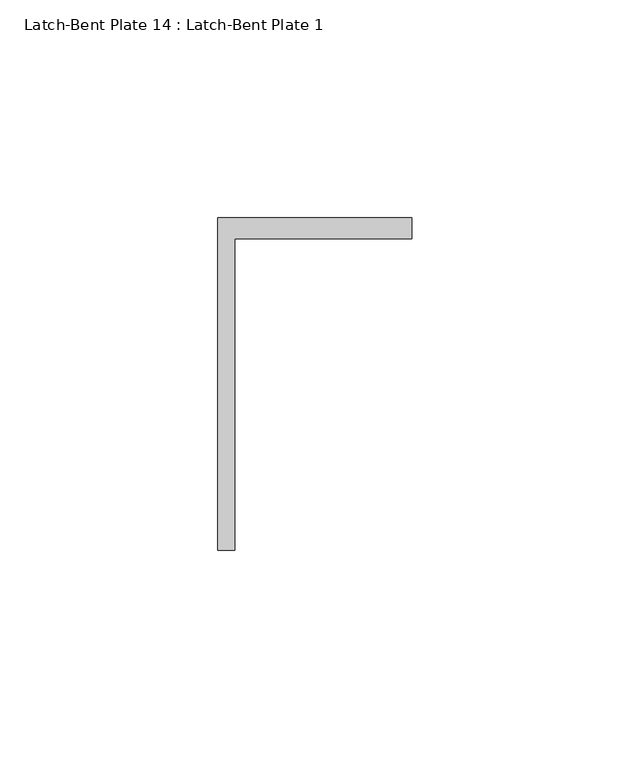
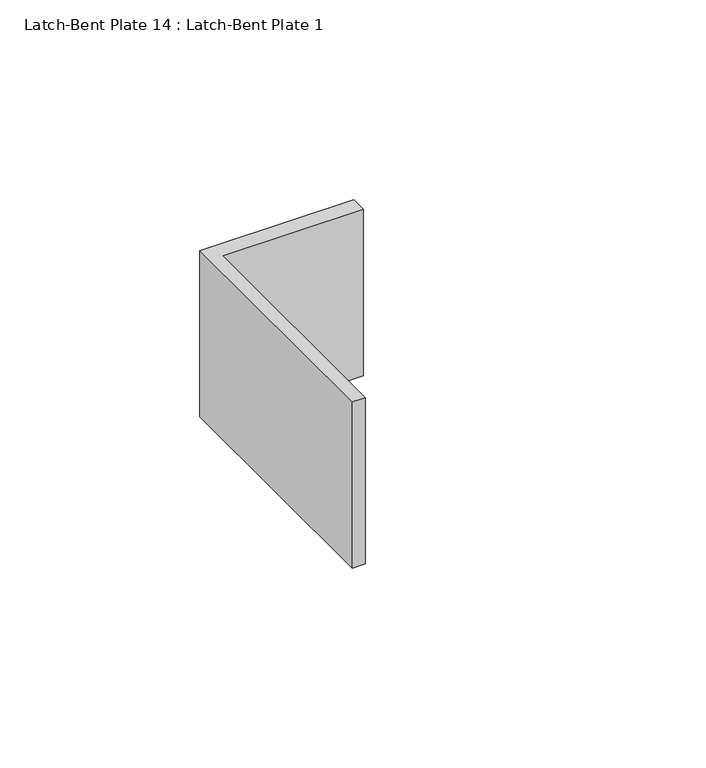
"""IFC4 building model written with IfcOpenShell, lengths in millimetres: proxy geometry, Latch-Bent Plate 14 : Latch-Bent Plate 1."""

from ifc_helpers import new_model, si_unit, frame, origin, place, context, project, spatial, polyline, outline, extrude, source, transform, mapped, element, save


def latch_bent_plate_14_latch_bent_plate_1_70bb7140(model_context):
    return source(origin(), model_context, "Body", "SweptSolid", [
        extrude(outline(polyline([(587327.0060739, -535207.9163841), (587366.6808739, -535207.9163841), (587366.6808739, -535212.6788841), (587326.1141748, -535212.6788841), (587326.1141748, -535284.1163841), (587322.2435739, -535284.1163841), (587322.2435739, -535207.9163841), (587327.0060739, -535207.9163841)])), frame((0.0, 0.0, 1041.4), z_axis=(0.0, 0.0, 1.0), x_axis=(1.0, 0.0, 0.0)), (0.0, 0.0, 1.0), 50.8),
    ])


if __name__ == "__main__":
    model = new_model("IFC4")
    model_context = context("Model", 3, world=origin())
    ifc_project = project(units=[si_unit("LENGTHUNIT", "METRE", prefix="MILLI")], contexts=[model_context])
    site = spatial("IfcSite", under=ifc_project)
    building = spatial("IfcBuilding", under=site)
    placement = place(None, origin())
    latch_bent_plate_14_latch_bent_plate_1_shape = latch_bent_plate_14_latch_bent_plate_1_70bb7140(model_context)
    element("IfcBuildingElementProxy", 1, Name="Latch-Bent Plate 14 : Latch-Bent Plate 1", ObjectType="Latch-Bent Plate 14 : Latch-Bent Plate 1", at=placement, inside=building, context=model_context, shape_type="MappedRepresentation", body=[
        mapped(latch_bent_plate_14_latch_bent_plate_1_shape, transform((0.0, 0.0, 0.0), x_axis=(1.0, 0.0, 0.0), y_axis=(0.0, 1.0, 0.0), z_axis=(0.0, 0.0, 1.0))),
    ])
    save(model, "model.ifc")

# Revit data of these elements
# Element 1 (IfcBuildingElementProxy, "Latch-Bent Plate 14 : Latch-Bent Plate 1")
#   Materials on its faces: "GALV. GATE LATCH"
# Materials
#   "GALV. GATE LATCH": class "Metal", colour RGB 189 187 185, transparency 0, Description = "Carbon steel", Cost = 0
